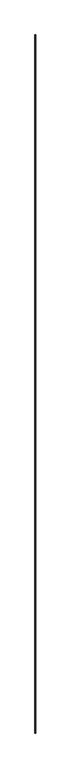
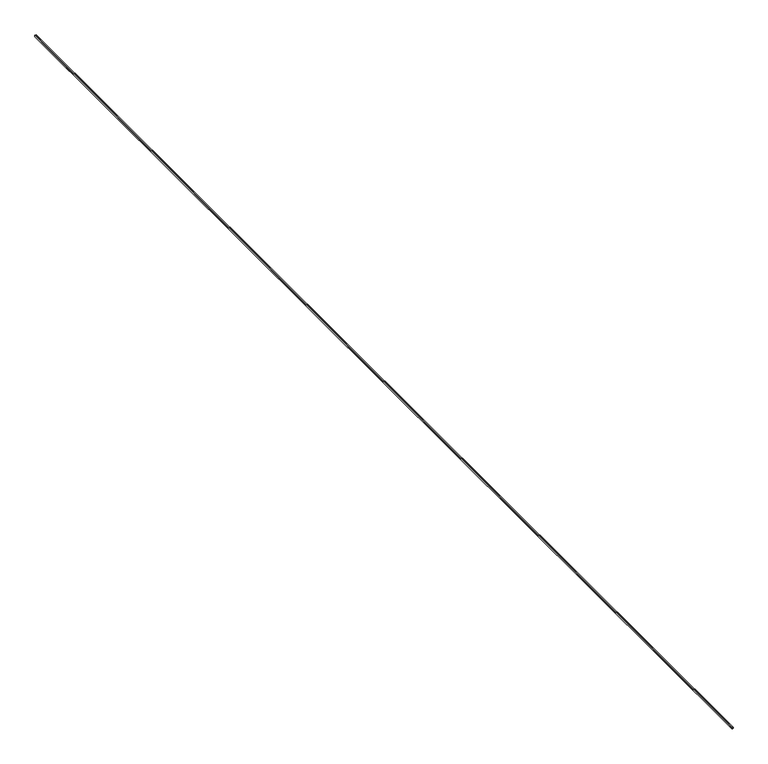
"""IFC4 building model written with IfcOpenShell, lengths in millimetres: proxy geometry, Inner panel:Inner panel:1:Inner panel:1 : Inner panel:Inner panel:300324:2:Inner panel:1:Inner panel:1 : Inner panel:Inner panel:300324:2 : Inner panel:Inner panel:1:Inner panel:1 : Inner panel:Inner panel:300324:300043:58 : Inner panel:Inner panel:1:Inner panel:1 : Inner panel:Inner panel:300324:2:Inner panel:1:Inner panel:1 : Inner panel:Inner panel:300324:2 : Inner panel:Inner panel:1:Inner panel:1 : Inner panel:Inner panel:300324:300043:308120."""

from ifc_helpers import new_model, si_unit, frame, origin, place, context, project, spatial, polyline, outline, extrude, source, transform, mapped, element, save


def generic_models_8aef5161(model_context):
    return source(origin(), model_context, "Body", "SweptSolid", [
        extrude(outline(polyline([(3913.3147263, 559487.6547197), (3910.9355406, 559487.7538524), (3911.5964255, 559503.61509), (3878.2878267, 559505.0029482), (3876.8999684, 559471.6943494), (3910.2085672, 559470.3064911), (3910.8694521, 559486.1677287), (3913.2486378, 559486.0685959), (3912.4886201, 559467.8281728), (3874.4216501, 559469.4142965), (3876.0077738, 559507.4812666), (3914.0747439, 559505.8951429), (3913.3147263, 559487.6547197)])), frame((0.0, -579337.5059673, 0.0), z_axis=(0.0, 1.0, 0.0), x_axis=(0.0, 0.0, 1.0)), (0.0, 0.0, 1.0), 33093.2895833),
    ])


if __name__ == "__main__":
    model = new_model("IFC4")
    model_context = context("Model", 3, world=origin())
    ifc_project = project(units=[si_unit("LENGTHUNIT", "METRE", prefix="MILLI")], contexts=[model_context])
    site = spatial("IfcSite", under=ifc_project)
    building = spatial("IfcBuilding", under=site)
    placement = place(None, origin())
    generic_models_shape = generic_models_8aef5161(model_context)
    element("IfcBuildingElementProxy", 1, Name="Inner panel:Inner panel:1:Inner panel:1 : Inner panel:Inner panel:300324:2:Inner panel:1:Inner panel:1 : Inner panel:Inner panel:300324:2 : Inner panel:Inner panel:1:Inner panel:1 : Inner panel:Inner panel:300324:300043:58 : Inner panel:Inner panel:1:Inner panel:1 : Inner panel:Inner panel:300324:2:Inner panel:1:Inner panel:1 : Inner panel:Inner panel:300324:2 : Inner panel:Inner panel:1:Inner panel:1 : Inner panel:Inner panel:300324:300043:308120", ObjectType="Inner panel:Inner panel:1:Inner panel:1 : Inner panel:Inner panel:300324:2:Inner panel:1:Inner panel:1 : Inner panel:Inner panel:300324:2 : Inner panel:Inner panel:1:Inner panel:1 : Inner panel:Inner panel:300324:300043:58 : Inner panel:Inner panel:1:Inner panel:1 : Inner panel:Inner panel:300324:2:Inner panel:1:Inner panel:1 : Inner panel:Inner panel:300324:2 : Inner panel:Inner panel:1:Inner panel:1 : Inner panel:Inner panel:300324:300043:308120", at=placement, inside=building, context=model_context, shape_type="MappedRepresentation", body=[
        mapped(generic_models_shape, transform((0.0, 0.0, 0.0), x_axis=(1.0, 0.0, 0.0), y_axis=(0.0, 1.0, 0.0), z_axis=(0.0, 0.0, 1.0))),
    ])
    save(model, "model.ifc")

# Revit data of these elements
# Type "Inner panel:Inner panel:1:Inner panel:1 : Inner panel:Inner panel:300324:2:Inner panel:1:Inner panel:1 : Inner panel:Inner panel:300324:2 : Inner panel:Inner panel:1:Inner panel:1 : Inner panel:Inner panel:300324:300043:58 : Inner panel:Inner panel:1:Inner panel:1 : Inner panel:Inner panel:300324:2:Inner panel:1:Inner panel:1 : Inner panel:Inner panel:300324:2 : Inner panel:Inner panel:1:Inner panel:1 : Inner panel:Inner panel:300324:300043:308120"
#   NameOverride = "Inner panel:Inner panel:1:Inner panel:1 : Inner panel:Inner panel:300324:2:Inner panel:1:Inner panel:1 : Inner panel:Inner panel:300324:2 : Inner panel:Inner panel:1:Inner panel:1 : Inner panel:Inner panel:300324:300043:308120"
#   ObjectTypeOverride = "Inner panel:1:Inner panel:1 : Inner panel:Inner panel:300324:2 : Inner panel:Inner panel:1:Inner panel:1 : Inner panel:Inner panel:300324:300043"
#   Reference = "Inner panel"
#   Tag = "308120"
# Element 1 (IfcBuildingElementProxy, "Inner panel:Inner panel:1:Inner panel:1 : Inner panel:Inner panel:300324:2:Inner panel:1:Inner panel:1 : Inner panel:Inner panel:300324:2 : Inner panel:Inner panel:1:Inner panel:1 : Inner panel:Inner panel:300324:300043:58 : Inner panel:Inner panel:1:Inner panel:1 : Inner panel:Inner panel:300324:2:Inner panel:1:Inner panel:1 : Inner panel:Inner panel:300324:2 : Inner panel:Inner panel:1:Inner panel:1 : Inner panel:Inner panel:300324:300043:308120")
#   Materials on its faces: "1 1/2\" X 1 1/2\" SPLIT-SEAM SQUARE TUBING (~24\" CANTILEVER FROM C.L. OF GLULAM)"
# Materials
#   "1 1/2\" X 1 1/2\" SPLIT-SEAM SQUARE TUBING (~24\" CANTILEVER FROM C.L. OF GLULAM)": class "Unassigned", colour RGB 202 201 200, transparency 0, Cost = 0
